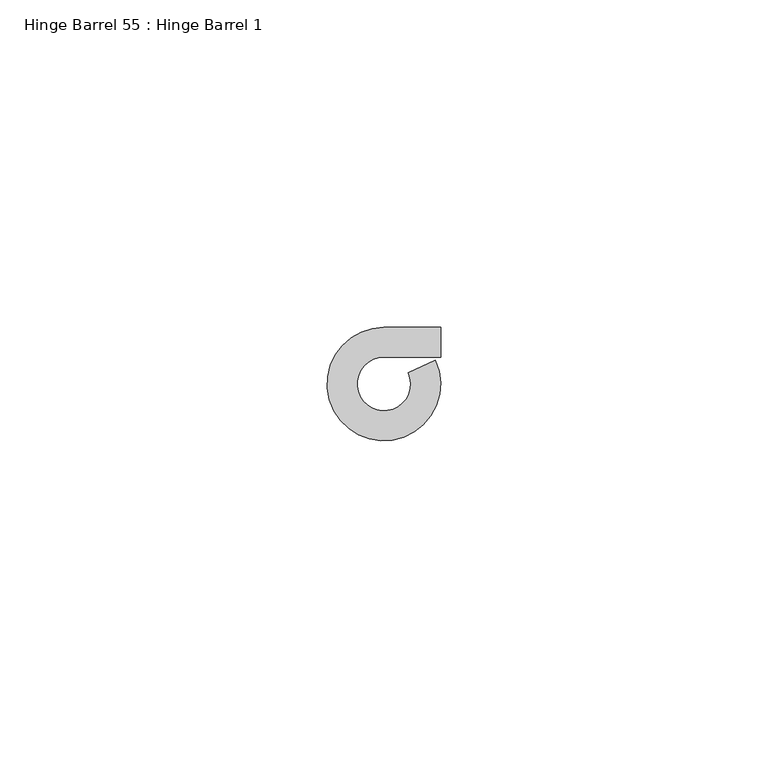
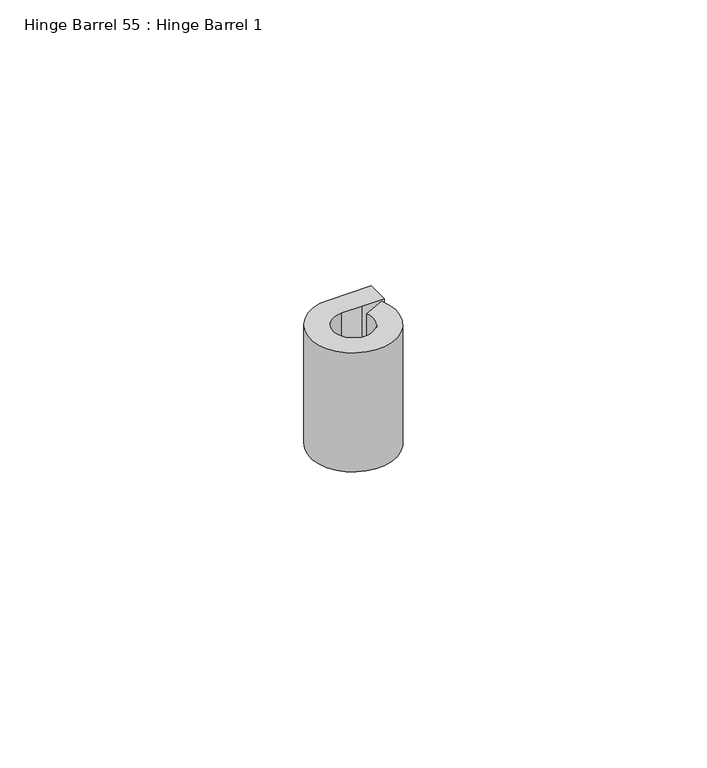
"""IFC4 building model written with IfcOpenShell, lengths in millimetres: proxy geometry, Hinge Barrel 55 : Hinge Barrel 1."""

from ifc_helpers import new_model, si_unit, point, frame, frame_2d, origin, place, context, project, spatial, polyline, circle_curve, trimmed, segment, composite_curve, outline, extrude, source, transform, mapped, element, save


def hinge_barrel_55_hinge_barrel_1_80958469(model_context):
    return source(origin(), model_context, "Body", "SweptSolid", [
        extrude(outline(composite_curve([segment(polyline([(587323.2214739, -536306.2758841), (587319.1320739, -536306.2758841)]), True, "CONTINUOUS"), segment(trimmed(circle_curve(frame_2d((587319.1320739, -536310.3652841)), 4.0894), [point((587319.1320739, -536306.2758841))], [point((587322.8436736, -536308.6485371))], True, "CARTESIAN"), True, "CONTINUOUS"), segment(polyline([(587322.8436736, -536308.6485371), (587326.986084, -536306.7325249)]), True, "CONTINUOUS"), segment(trimmed(circle_curve(frame_2d((587319.1320739, -536310.3652841)), 8.6534625), [point((587326.986084, -536306.7325249))], [point((587319.1320739, -536301.7118216))], False, "CARTESIAN"), True, "CONTINUOUS"), segment(polyline([(587319.1320739, -536301.7118216), (587327.7934739, -536301.7118216), (587327.7934739, -536306.2758841), (587323.2214739, -536306.2758841)]), True, "CONTINUOUS")], self_intersect=False)), frame((0.0, 0.0, 311.15), z_axis=(0.0, 0.0, 1.0), x_axis=(1.0, 0.0, 0.0)), (0.0, 0.0, 1.0), 25.4),
    ])


if __name__ == "__main__":
    model = new_model("IFC4")
    model_context = context("Model", 3, world=origin())
    ifc_project = project(units=[si_unit("LENGTHUNIT", "METRE", prefix="MILLI")], contexts=[model_context])
    site = spatial("IfcSite", under=ifc_project)
    building = spatial("IfcBuilding", under=site)
    placement = place(None, origin())
    hinge_barrel_55_hinge_barrel_1_shape = hinge_barrel_55_hinge_barrel_1_80958469(model_context)
    element("IfcBuildingElementProxy", 1, Name="Hinge Barrel 55 : Hinge Barrel 1", ObjectType="Hinge Barrel 55 : Hinge Barrel 1", at=placement, inside=building, context=model_context, shape_type="MappedRepresentation", body=[
        mapped(hinge_barrel_55_hinge_barrel_1_shape, transform((0.0, 0.0, 0.0), x_axis=(1.0, 0.0, 0.0), y_axis=(0.0, 1.0, 0.0), z_axis=(0.0, 0.0, 1.0))),
    ])
    save(model, "model.ifc")

# Revit data of these elements
# Element 1 (IfcBuildingElementProxy, "Hinge Barrel 55 : Hinge Barrel 1")
#   Materials on its faces: "6\"X6\" WELD-ON STL BUTT HINGE"
# Materials
#   "6\"X6\" WELD-ON STL BUTT HINGE": class "Metal", colour RGB 189 187 185, transparency 0, Description = "Carbon steel", Cost = 0
